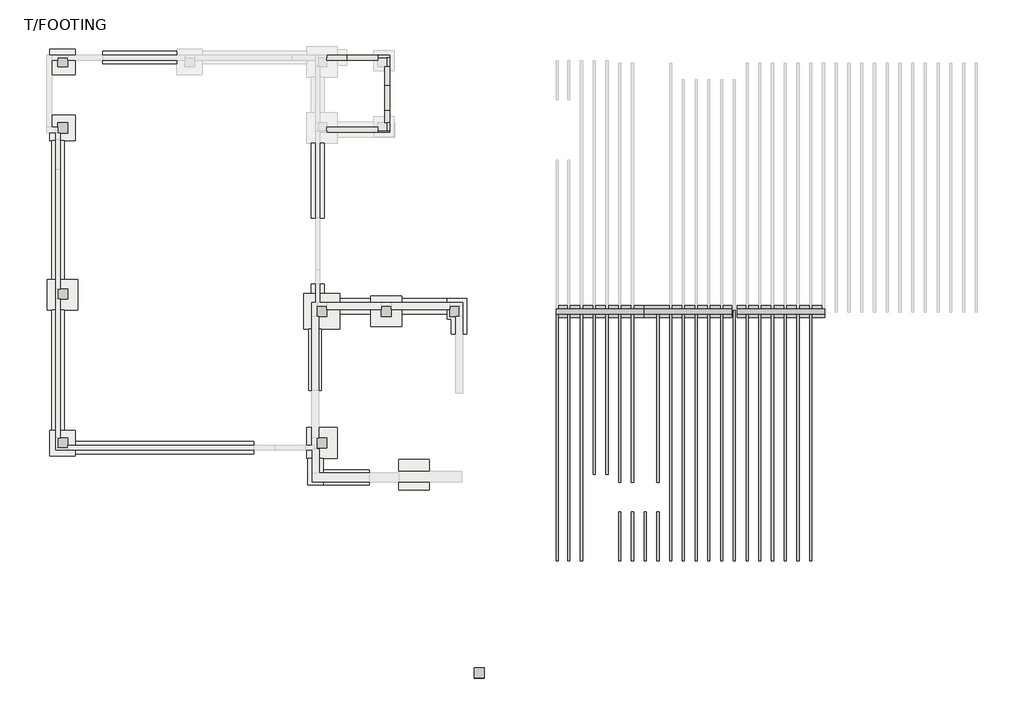
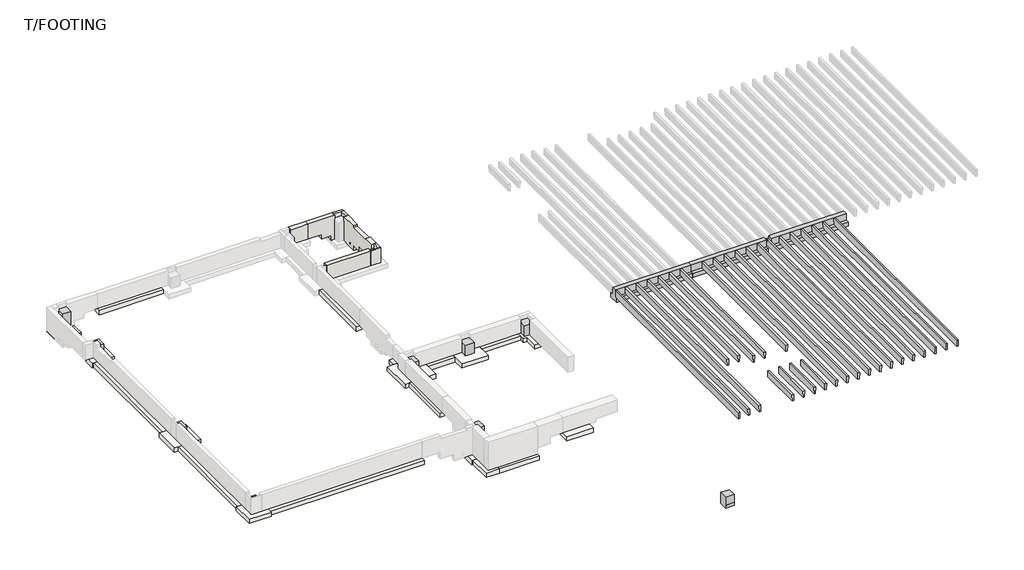
# One storey, part 2 of 3: 27 beams, 11 footings, 9 columns, 9 slabs, 8 walls.
"""IFC4 building model written with IfcOpenShell, lengths in millimetres."""

import ifcopenshell
import ifcopenshell.guid

model = None  # the IFC model being written
_history = None  # IfcOwnerHistory: only IFC2X3 demands one
_inside = {}  # id of a spatial element -> (the spatial element, [elements in it])
_under = {}  # id of a project, library or spatial element -> (it, [spatial elements below it])
_declared = {}  # id of a project -> (the project, [libraries it declares])
_typed = {}  # id of a type object -> (the type object, [elements of that type])
_made_of = {}  # id of a material, layer set ... -> (it, [elements and type objects made of it])


def new_model(schema):
    """Start an empty IFC model of exactly this schema.

    Asked for "IFC4X3", IfcOpenShell would pick the latest addendum, in which some entities
    have other attributes; the version numbers below select the first issue.
    IFC2X3 requires an IfcOwnerHistory on every rooted entity: one is made here for all.
    """
    global model, _history
    if schema == "IFC4X3":
        model = ifcopenshell.file(schema_version=(4, 3, 0, 0))
    else:
        model = ifcopenshell.file(schema=schema)
    _inside.clear()
    _under.clear()
    _declared.clear()
    _typed.clear()
    _made_of.clear()
    _history = None
    if model.schema == "IFC2X3":
        org = make("IfcOrganization", Name="unknown")
        user = make(
            "IfcPersonAndOrganization",
            ThePerson=make("IfcPerson", FamilyName="unknown"),
            TheOrganization=org,
        )
        app = make(
            "IfcApplication",
            ApplicationDeveloper=org,
            Version="unknown",
            ApplicationFullName="unknown",
            ApplicationIdentifier="unknown",
        )
        _history = make(
            "IfcOwnerHistory",
            OwningUser=user,
            OwningApplication=app,
            ChangeAction="ADDED",
            CreationDate=0,
        )
    return model


def make(cls, **values):
    """One entity of the class cls with the attributes given. An attribute that is None is left unset."""
    return model.create_entity(
        cls, **{name: value for name, value in values.items() if value is not None}
    )


def rooted(cls, **values):
    """An entity with a GlobalId (a new one), such as an element, a storey or a relation."""
    return make(cls, GlobalId=ifcopenshell.guid.new(), OwnerHistory=_history, **values)


def si_unit(unit_type, name, prefix=None):
    """IfcSIUnit, for example si_unit("LENGTHUNIT", "METRE", prefix="MILLI")."""
    return make("IfcSIUnit", UnitType=unit_type, Prefix=prefix, Name=name)


def assignment(units):
    """IfcUnitAssignment: the units of a project."""
    return None if units is None else make("IfcUnitAssignment", Units=units)


def point(xyz):
    """IfcCartesianPoint."""
    return None if xyz is None else make("IfcCartesianPoint", Coordinates=xyz)


def direction(xyz):
    """IfcDirection."""
    return None if xyz is None else make("IfcDirection", DirectionRatios=xyz)


def frame(location, z_axis=None, x_axis=None):
    """IfcAxis2Placement3D, a coordinate frame: its origin and axes. An axis left out is left unset."""
    return make(
        "IfcAxis2Placement3D",
        Location=point(location),
        Axis=direction(z_axis),
        RefDirection=direction(x_axis),
    )


def origin():
    """The frame at (0, 0, 0) with its axes left unset."""
    return frame((0.0, 0.0, 0.0))


def place(relative_to, where):
    """IfcLocalPlacement: puts the frame where relative to a parent placement (None: the world)."""
    return make(
        "IfcLocalPlacement", PlacementRelTo=relative_to, RelativePlacement=where
    )


def context(
    kind, dimensions, precision=None, world=None, true_north=None, identifier=None
):
    """IfcGeometricRepresentationContext, for example the 3D "Model" context."""
    return make(
        "IfcGeometricRepresentationContext",
        ContextIdentifier=identifier,
        ContextType=kind,
        CoordinateSpaceDimension=dimensions,
        Precision=precision,
        WorldCoordinateSystem=world,
        TrueNorth=true_north,
    )


def project(units=None, contexts=None):
    """IfcProject with its units and contexts."""
    return rooted(
        "IfcProject",
        Name="project",
        RepresentationContexts=contexts,
        UnitsInContext=assignment(units),
    )


def spatial(cls, under=None, at=None, **own):
    """A site, building, storey or space (cls), placed at a placement, below another one or the project."""
    s = rooted(cls, ObjectPlacement=at, **own)
    if under is not None:
        _under.setdefault(under.id(), (under, []))[1].append(s)
    return s


def polyline(points):
    """IfcPolyline through the points."""
    return make("IfcPolyline", Points=[point(p) for p in points])


def circle_curve(where, radius):
    """IfcCircle in the frame where."""
    return make("IfcCircle", Position=where, Radius=radius)


def outline(outer, holes=None, kind="AREA"):
    """IfcArbitraryClosedProfileDef: a profile drawn as a closed curve; with holes, ...WithVoids."""
    if holes is None:
        return make("IfcArbitraryClosedProfileDef", ProfileType=kind, OuterCurve=outer)
    return make(
        "IfcArbitraryProfileDefWithVoids",
        ProfileType=kind,
        OuterCurve=outer,
        InnerCurves=holes,
    )


def extrude(swept, where, along, depth):
    """IfcExtrudedAreaSolid: the profile swept, set in the frame where, extruded along a direction by depth."""
    return make(
        "IfcExtrudedAreaSolid",
        SweptArea=swept,
        Position=where,
        ExtrudedDirection=direction(along),
        Depth=depth,
    )


def faces_of(points, faces, orient=None, outer=None):
    """IfcFace entities. A face is a list of loops; a loop is a list of indices into points, from 0.

    orient and outer hold one flag for each loop. By default every Orientation is true, the
    first loop of a face is its IfcFaceOuterBound and the others are IfcFaceBound.
    """
    made = []
    for i, loops in enumerate(faces):
        bounds = []
        for j, loop in enumerate(loops):
            is_outer = j == 0 if outer is None else outer[i][j]
            bounds.append(
                make(
                    "IfcFaceOuterBound" if is_outer else "IfcFaceBound",
                    Bound=make("IfcPolyLoop", Polygon=[points[k] for k in loop]),
                    Orientation=True if orient is None else orient[i][j],
                )
            )
        made.append(make("IfcFace", Bounds=bounds))
    return made


def faceted_brep(points, faces, orient=None, outer=None, voids=None):
    """IfcFacetedBrep: a solid bounded by flat faces; with voids (closed shells), ...WithVoids."""
    shared = [point(p) for p in points]
    hull = make("IfcClosedShell", CfsFaces=faces_of(shared, faces, orient, outer))
    if voids is None:
        return make("IfcFacetedBrep", Outer=hull)
    return make(
        "IfcFacetedBrepWithVoids",
        Outer=hull,
        Voids=[
            make(cls, CfsFaces=faces_of(shared, fs, o, b)) for cls, fs, o, b in voids
        ],
    )


def shape(context_of_items, identifier, shape_type, items):
    """IfcShapeRepresentation: the items that make up one representation, for example the "Body"."""
    return make(
        "IfcShapeRepresentation",
        ContextOfItems=context_of_items,
        RepresentationIdentifier=identifier,
        RepresentationType=shape_type,
        Items=items,
    )


def source(mapping_origin, context_of_items, identifier, shape_type, items):
    """IfcRepresentationMap: a shape defined once, which mapped items show again and again."""
    return make(
        "IfcRepresentationMap",
        MappingOrigin=mapping_origin,
        MappedRepresentation=shape(context_of_items, identifier, shape_type, items),
    )


def transform(
    local_origin,
    x_axis=None,
    y_axis=None,
    z_axis=None,
    scale=None,
    scale2=None,
    scale3=None,
    uniform=True,
):
    """IfcCartesianTransformationOperator3D, or its non-uniform kind. x_axis, y_axis, z_axis: its Axis1, 2, 3."""
    if uniform:
        return make(
            "IfcCartesianTransformationOperator3D",
            Axis1=direction(x_axis),
            Axis2=direction(y_axis),
            LocalOrigin=point(local_origin),
            Scale=scale,
            Axis3=direction(z_axis),
        )
    return make(
        "IfcCartesianTransformationOperator3DnonUniform",
        Axis1=direction(x_axis),
        Axis2=direction(y_axis),
        LocalOrigin=point(local_origin),
        Scale=scale,
        Axis3=direction(z_axis),
        Scale2=scale2,
        Scale3=scale3,
    )


def mapped(mapping_source, mapping_target):
    """IfcMappedItem: shows the shape of a source again, moved by a transform."""
    return make(
        "IfcMappedItem", MappingSource=mapping_source, MappingTarget=mapping_target
    )


def made_of(thing, what):
    """Note that an element or type object is made of a material, layer set ...; save() writes the relation."""
    if what is not None:
        _made_of.setdefault(what.id(), (what, []))[1].append(thing)
    return thing


def element(
    cls,
    number,
    at=None,
    inside=None,
    cuts=None,
    type_object=None,
    material=None,
    context=None,
    identifier="Body",
    shape_type=None,
    held_by="IfcProductDefinitionShape",
    body=None,
    shapes=None,
    **own,
):
    """One element of the class cls, such as IfcWall. Its Tag is "e" and its number.

    at: its placement. inside: the storey or other place that contains it. cuts: it is an
    opening in that element (IfcRelVoidsElement). A single representation is given by context,
    identifier, shape_type and body (its items); several are given by shapes. held_by: the class
    of the entity that holds the representations. save() writes the other relations.
    """
    e = rooted(cls, Tag="e%d" % number, ObjectPlacement=at, **own)
    if body is not None:
        shapes = [shape(context, identifier, shape_type, body)]
    if shapes is not None:
        e.Representation = make(held_by, Representations=shapes)
    if inside is not None:
        _inside.setdefault(inside.id(), (inside, []))[1].append(e)
    if cuts is not None:
        rooted(
            "IfcRelVoidsElement", RelatingBuildingElement=cuts, RelatedOpeningElement=e
        )
    if type_object is not None:
        _typed.setdefault(type_object.id(), (type_object, []))[1].append(e)
    return made_of(e, material)


def aggregate(whole, parts):
    """IfcRelAggregates: a whole, such as a stair, and the parts it consists of."""
    return rooted("IfcRelAggregates", RelatingObject=whole, RelatedObjects=parts)


def save(model, path):
    """Write the relations noted so far, then the file.

    IfcRelAggregates (storeys below a building ...), IfcRelContainedInSpatialStructure (elements
    in a storey), IfcRelDefinesByType, IfcRelAssociatesMaterial and IfcRelDeclares: one each for
    every whole, place, type object, material and project.
    """
    for whole, parts in _under.values():
        aggregate(whole, parts)
    for where, things in _inside.values():
        rooted(
            "IfcRelContainedInSpatialStructure",
            RelatedElements=things,
            RelatingStructure=where,
        )
    for kind, things in _typed.values():
        rooted("IfcRelDefinesByType", RelatedObjects=things, RelatingType=kind)
    for what, things in _made_of.values():
        rooted("IfcRelAssociatesMaterial", RelatedObjects=things, RelatingMaterial=what)
    for by, libraries in _declared.values():
        rooted("IfcRelDeclares", RelatingContext=by, RelatedDefinitions=libraries)
    model.write(path)


def plane_surface(at):
    """IfcPlane: the flat surface through the origin of the frame at, square to its z axis."""
    return make("IfcPlane", Position=at)


def revolved_surface(curve, axis_point, axis_direction):
    """IfcSurfaceOfRevolution: the curve turned about the line through axis_point along axis_direction."""
    return make(
        "IfcSurfaceOfRevolution",
        SweptCurve=make("IfcArbitraryOpenProfileDef", ProfileType="CURVE", Curve=curve),
        AxisPosition=make("IfcAxis1Placement", Location=point(axis_point), Axis=direction(axis_direction)),
    )


def advanced_brep(points, edges, surfaces, faces):
    """IfcAdvancedBrep: a solid bounded by faces that lie on surfaces and meet in shared edges.

    An edge is (start, end): straight between two places in points (the first is 0);
    or (start, end, curve); or (start, end, curve, False) where it runs against its curve.
    A face is (place in surfaces, loops), or (place, loops, False) where it looks against
    its surface's normal. A loop lists edges by number (the first is 1), with a minus sign
    where the edge is run from its end to its start. The first loop is the outer one.
    """
    corners = [point(p) for p in points]
    vertices = [make("IfcVertexPoint", VertexGeometry=c) for c in corners]
    made = []
    for start, end, *more in edges:
        made.append(
            make(
                "IfcEdgeCurve",
                EdgeStart=vertices[start],
                EdgeEnd=vertices[end],
                EdgeGeometry=more[0] if more else make("IfcPolyline", Points=[corners[start], corners[end]]),
                SameSense=more[1] if len(more) > 1 else True,
            )
        )
    hull = []
    for where, loops, *sense in faces:
        bounds = []
        for j, loop in enumerate(loops):
            ring = [make("IfcOrientedEdge", EdgeElement=made[abs(k) - 1], Orientation=k > 0) for k in loop]
            bounds.append(
                make(
                    "IfcFaceOuterBound" if j == 0 else "IfcFaceBound",
                    Bound=make("IfcEdgeLoop", EdgeList=ring),
                    Orientation=True,
                )
            )
        hull.append(make("IfcAdvancedFace", Bounds=bounds, FaceSurface=surfaces[where], SameSense=sense[0] if sense else True))
    return make("IfcAdvancedBrep", Outer=make("IfcClosedShell", CfsFaces=hull))


def precast_cone_shaped_beam_double_t_64f85e83(model_context):
    return source(origin(), model_context, "Body", "SweptSolid", [
        extrude(outline(polyline([(-50.8, -228.6), (-63.5, 228.6), (63.5, 228.6), (50.8, -228.6), (-50.8, -228.6)])), frame((-7391.4, 0.0, 0.0), z_axis=(1.0, 0.0, 0.0), x_axis=(0.0, 1.0, 0.0)), (0.0, 0.0, 1.0), 14770.1),
    ])


def precast_cone_shaped_beam_double_t_17914b82(model_context):
    return source(origin(), model_context, "Body", "SweptSolid", [
        extrude(outline(polyline([(-50.8, -228.6), (-63.5, 228.6), (63.5, 228.6), (50.8, -228.6), (-50.8, -228.6)])), frame((-7594.6, 0.0, 0.0), z_axis=(1.0, 0.0, 0.0), x_axis=(0.0, 1.0, 0.0)), (0.0, 0.0, 1.0), 14973.3),
    ])


def precast_cone_shaped_beam_double_t_a1b90a55(model_context):
    return source(origin(), model_context, "Body", "SweptSolid", [
        extrude(outline(polyline([(-50.8, -228.6), (-63.5, 228.6), (63.5, 228.6), (50.8, -228.6), (-50.8, -228.6)])), frame((-4891.88125, 0.0, 0.0), z_axis=(1.0, 0.0, 0.0), x_axis=(0.0, 1.0, 0.0)), (0.0, 0.0, 1.0), 10083.8),
    ])


def precast_cone_shaped_beam_double_t_8ba99103(model_context):
    return source(origin(), model_context, "Body", "SweptSolid", [
        extrude(outline(polyline([(50.8, -228.6), (-50.8, -228.6), (-63.5, 228.6), (63.5, 228.6), (50.8, -228.6)])), frame((-1610.51875, 0.0, 0.0), z_axis=(1.0, 0.0, 0.0), x_axis=(0.0, 1.0, 0.0)), (0.0, 0.0, 1.0), 2908.3),
    ])


def precast_cone_shaped_beam_double_t_5ff23cd5(model_context):
    return source(origin(), model_context, "Body", "SweptSolid", [
        extrude(outline(polyline([(-50.8, -228.6), (-63.5, 228.6), (63.5, 228.6), (50.8, -228.6), (-50.8, -228.6)])), frame((-4660.9, 0.0, 0.0), z_axis=(1.0, 0.0, 0.0), x_axis=(0.0, 1.0, 0.0)), (0.0, 0.0, 1.0), 9601.2),
    ])


def precast_inverted_tee_20_12x28_77df7164(model_context):
    return source(origin(), model_context, "Body", "SweptSolid", [
        extrude(outline(polyline([(-355.6, -406.4), (-355.6, -101.6), (-152.4, -101.6), (-152.4, 406.4), (152.4, 406.4), (152.4, -101.6), (355.6, -101.6), (355.6, -406.4), (-355.6, -406.4)])), frame((-2728.5280327, 0.0, 0.0), z_axis=(1.0, 0.0, 0.0), x_axis=(0.0, 1.0, 0.0)), (0.0, 0.0, 1.0), 5228.4560654),
    ])


def precast_inverted_tee_20_12x28_0a739a6f(model_context):
    return source(origin(), model_context, "Body", "SweptSolid", [
        extrude(outline(polyline([(355.6, -406.4), (-355.6, -406.4), (-355.6, -101.6), (-152.4, -101.6), (-152.4, 406.4), (152.4, 406.4), (152.4, -101.6), (355.6, -101.6), (355.6, -406.4)])), frame((-2692.4, 0.0, 0.0), z_axis=(1.0, 0.0, 0.0), x_axis=(0.0, 1.0, 0.0)), (0.0, 0.0, 1.0), 5245.1),
    ])


def precast_inverted_tee_20_12x28_b7649b98(model_context):
    return source(origin(), model_context, "Body", "SweptSolid", [
        extrude(outline(polyline([(355.6, -406.4), (-355.6, -406.4), (-355.6, -101.6), (-152.4, -101.6), (-152.4, 406.4), (152.4, 406.4), (152.4, -101.6), (355.6, -101.6), (355.6, -406.4)])), frame((-2730.5, 0.0, 0.0), z_axis=(1.0, 0.0, 0.0), x_axis=(0.0, 1.0, 0.0)), (0.0, 0.0, 1.0), 5232.4),
    ])


model = new_model("IFC4")

# Units and contexts
model_context = context("Model", 3, world=origin())
ifc_project = project(units=[si_unit("LENGTHUNIT", "METRE", prefix="MILLI")], contexts=[model_context])

# Site, building, storey
site = spatial("IfcSite", under=ifc_project)
building = spatial("IfcBuilding", under=site)
storey = spatial("IfcBuildingStorey", under=building, Name="T/FOOTING", Elevation=-1092.2)

# Beams
placement = place(None, origin())
precast_cone_shaped_beam_double_t_shape = precast_cone_shaped_beam_double_t_64f85e83(model_context)
element("IfcBeam", 1, ObjectType="Precast-Cone Shaped Beam : DOUBLE_T", at=placement, inside=storey, context=model_context, shape_type="MappedRepresentation", body=[
    mapped(precast_cone_shaped_beam_double_t_shape, transform((-28033.5909443, -9707.8231529, -279.4), x_axis=(0.0, -1.0, 0.0), y_axis=(1.0, 0.0, 0.0), z_axis=(0.0, 0.0, 1.0))),
])
element("IfcBeam", 2, ObjectType="Precast-Cone Shaped Beam : DOUBLE_T", at=placement, inside=storey, context=model_context, shape_type="MappedRepresentation", body=[
    mapped(precast_cone_shaped_beam_double_t_shape, transform((-27271.5909443, -9707.8231529, -279.4), x_axis=(0.0, -1.0, 0.0), y_axis=(1.0, 0.0, 0.0), z_axis=(0.0, 0.0, 1.0))),
])
element("IfcBeam", 3, ObjectType="Precast-Cone Shaped Beam : DOUBLE_T", at=placement, inside=storey, context=model_context, shape_type="MappedRepresentation", body=[
    mapped(precast_cone_shaped_beam_double_t_shape, transform((-26509.5909443, -9707.8231529, -279.4), x_axis=(0.0, -1.0, 0.0), y_axis=(1.0, 0.0, 0.0), z_axis=(0.0, 0.0, 1.0))),
])
element("IfcBeam", 4, ObjectType="Precast-Cone Shaped Beam : DOUBLE_T", at=placement, inside=storey, context=model_context, shape_type="MappedRepresentation", body=[
    mapped(precast_cone_shaped_beam_double_t_shape, transform((-25747.5909443, -9707.8231529, -279.4), x_axis=(0.0, -1.0, 0.0), y_axis=(1.0, 0.0, 0.0), z_axis=(0.0, 0.0, 1.0))),
])
element("IfcBeam", 5, ObjectType="Precast-Cone Shaped Beam : DOUBLE_T", at=placement, inside=storey, context=model_context, shape_type="MappedRepresentation", body=[
    mapped(precast_cone_shaped_beam_double_t_shape, transform((-24985.5909443, -9707.8231529, -279.4), x_axis=(0.0, -1.0, 0.0), y_axis=(1.0, 0.0, 0.0), z_axis=(0.0, 0.0, 1.0))),
])
element("IfcBeam", 6, ObjectType="Precast-Cone Shaped Beam : DOUBLE_T", at=placement, inside=storey, context=model_context, shape_type="MappedRepresentation", body=[
    mapped(precast_cone_shaped_beam_double_t_shape, transform((-23461.5909443, -9707.8231529, -279.4), x_axis=(0.0, -1.0, 0.0), y_axis=(1.0, 0.0, 0.0), z_axis=(0.0, 0.0, 1.0))),
])
element("IfcBeam", 7, ObjectType="Precast-Cone Shaped Beam : DOUBLE_T", at=placement, inside=storey, context=model_context, shape_type="MappedRepresentation", body=[
    mapped(precast_cone_shaped_beam_double_t_shape, transform((-22699.5909443, -9707.8231529, -279.4), x_axis=(0.0, -1.0, 0.0), y_axis=(1.0, 0.0, 0.0), z_axis=(0.0, 0.0, 1.0))),
])
element("IfcBeam", 8, ObjectType="Precast-Cone Shaped Beam : DOUBLE_T", at=placement, inside=storey, context=model_context, shape_type="MappedRepresentation", body=[
    mapped(precast_cone_shaped_beam_double_t_shape, transform((-21940.4905844, -9707.8231529, -279.4), x_axis=(0.0, -1.0, 0.0), y_axis=(1.0, 0.0, 0.0), z_axis=(0.0, 0.0, 1.0))),
])
element("IfcBeam", 9, ObjectType="Precast-Cone Shaped Beam : DOUBLE_T", at=placement, inside=storey, context=model_context, shape_type="MappedRepresentation", body=[
    mapped(precast_cone_shaped_beam_double_t_shape, transform((-21179.5348789, -9707.8231529, -279.4), x_axis=(0.0, -1.0, 0.0), y_axis=(1.0, 0.0, 0.0), z_axis=(0.0, 0.0, 1.0))),
])
element("IfcBeam", 10, ObjectType="Precast-Cone Shaped Beam : DOUBLE_T", at=placement, inside=storey, context=model_context, shape_type="MappedRepresentation", body=[
    mapped(precast_cone_shaped_beam_double_t_shape, transform((-20417.5348789, -9707.8231529, -279.4), x_axis=(0.0, -1.0, 0.0), y_axis=(1.0, 0.0, 0.0), z_axis=(0.0, 0.0, 1.0))),
])
element("IfcBeam", 11, ObjectType="Precast-Cone Shaped Beam : DOUBLE_T", at=placement, inside=storey, context=model_context, shape_type="MappedRepresentation", body=[
    mapped(precast_cone_shaped_beam_double_t_shape, transform((-19655.5348789, -9707.8231529, -279.4), x_axis=(0.0, -1.0, 0.0), y_axis=(1.0, 0.0, 0.0), z_axis=(0.0, 0.0, 1.0))),
])
element("IfcBeam", 12, ObjectType="Precast-Cone Shaped Beam : DOUBLE_T", at=placement, inside=storey, context=model_context, shape_type="MappedRepresentation", body=[
    mapped(precast_cone_shaped_beam_double_t_shape, transform((-33367.5909443, -9707.8231529, -279.4), x_axis=(0.0, -1.0, 0.0), y_axis=(1.0, 0.0, 0.0), z_axis=(0.0, 0.0, 1.0))),
])
element("IfcBeam", 13, ObjectType="Precast-Cone Shaped Beam : DOUBLE_T", at=placement, inside=storey, context=model_context, shape_type="MappedRepresentation", body=[
    mapped(precast_cone_shaped_beam_double_t_shape, transform((-34129.5909443, -9707.8231529, -279.4), x_axis=(0.0, -1.0, 0.0), y_axis=(1.0, 0.0, 0.0), z_axis=(0.0, 0.0, 1.0))),
])
element("IfcBeam", 14, ObjectType="Precast-Cone Shaped Beam : DOUBLE_T", at=placement, inside=storey, context=model_context, shape_type="MappedRepresentation", body=[
    mapped(precast_cone_shaped_beam_double_t_shape, transform((-34815.3909443, -9707.8231529, -279.4), x_axis=(0.0, -1.0, 0.0), y_axis=(1.0, 0.0, 0.0), z_axis=(0.0, 0.0, 1.0))),
])
precast_cone_shaped_beam_double_t_2_shape = precast_cone_shaped_beam_double_t_17914b82(model_context)
element("IfcBeam", 15, ObjectType="Precast-Cone Shaped Beam : DOUBLE_T", at=placement, inside=storey, context=model_context, shape_type="MappedRepresentation", body=[
    mapped(precast_cone_shaped_beam_double_t_2_shape, transform((-24223.5909443, -9707.8231529, -279.4), x_axis=(0.0, -1.0, 0.0), y_axis=(1.0, 0.0, 0.0), z_axis=(0.0, 0.0, 1.0))),
])
precast_cone_shaped_beam_double_t_3_shape = precast_cone_shaped_beam_double_t_a1b90a55(model_context)
element("IfcBeam", 16, ObjectType="Precast-Cone Shaped Beam : DOUBLE_T", at=placement, inside=storey, context=model_context, shape_type="MappedRepresentation", body=[
    mapped(precast_cone_shaped_beam_double_t_3_shape, transform((-28795.5909443, -7208.3044029, -279.4), x_axis=(0.0, -1.0, 0.0), y_axis=(1.0, 0.0, 0.0), z_axis=(0.0, 0.0, 1.0))),
])
element("IfcBeam", 17, ObjectType="Precast-Cone Shaped Beam : DOUBLE_T", at=placement, inside=storey, context=model_context, shape_type="MappedRepresentation", body=[
    mapped(precast_cone_shaped_beam_double_t_3_shape, transform((-30319.5909443, -7208.3044029, -279.4), x_axis=(0.0, -1.0, 0.0), y_axis=(1.0, 0.0, 0.0), z_axis=(0.0, 0.0, 1.0))),
])
element("IfcBeam", 18, ObjectType="Precast-Cone Shaped Beam : DOUBLE_T", at=placement, inside=storey, context=model_context, shape_type="MappedRepresentation", body=[
    mapped(precast_cone_shaped_beam_double_t_3_shape, transform((-31081.5909443, -7208.3044029, -279.4), x_axis=(0.0, -1.0, 0.0), y_axis=(1.0, 0.0, 0.0), z_axis=(0.0, 0.0, 1.0))),
])
precast_cone_shaped_beam_double_t_4_shape = precast_cone_shaped_beam_double_t_8ba99103(model_context)
element("IfcBeam", 19, ObjectType="Precast-Cone Shaped Beam : DOUBLE_T", at=placement, inside=storey, context=model_context, shape_type="MappedRepresentation", body=[
    mapped(precast_cone_shaped_beam_double_t_4_shape, transform((-28795.5909443, -15788.7419029, -279.4), x_axis=(0.0, -1.0, 0.0), y_axis=(1.0, 0.0, 0.0), z_axis=(0.0, 0.0, 1.0))),
])
element("IfcBeam", 20, ObjectType="Precast-Cone Shaped Beam : DOUBLE_T", at=placement, inside=storey, context=model_context, shape_type="MappedRepresentation", body=[
    mapped(precast_cone_shaped_beam_double_t_4_shape, transform((-30319.5909443, -15788.7419029, -279.4), x_axis=(0.0, -1.0, 0.0), y_axis=(1.0, 0.0, 0.0), z_axis=(0.0, 0.0, 1.0))),
])
element("IfcBeam", 21, ObjectType="Precast-Cone Shaped Beam : DOUBLE_T", at=placement, inside=storey, context=model_context, shape_type="MappedRepresentation", body=[
    mapped(precast_cone_shaped_beam_double_t_4_shape, transform((-31081.5909443, -15788.7419029, -279.4), x_axis=(0.0, -1.0, 0.0), y_axis=(1.0, 0.0, 0.0), z_axis=(0.0, 0.0, 1.0))),
])
element("IfcBeam", 22, ObjectType="Precast-Cone Shaped Beam : DOUBLE_T", at=placement, inside=storey, context=model_context, shape_type="MappedRepresentation", body=[
    mapped(precast_cone_shaped_beam_double_t_4_shape, transform((-29557.5909443, -15788.7419029, -279.4), x_axis=(0.0, -1.0, 0.0), y_axis=(1.0, 0.0, 0.0), z_axis=(0.0, 0.0, 1.0))),
])
precast_cone_shaped_beam_double_t_5_shape = precast_cone_shaped_beam_double_t_5ff23cd5(model_context)
element("IfcBeam", 23, ObjectType="Precast-Cone Shaped Beam : DOUBLE_T", at=placement, inside=storey, context=model_context, shape_type="MappedRepresentation", body=[
    mapped(precast_cone_shaped_beam_double_t_5_shape, transform((-31843.5909443, -6977.3231529, -279.4), x_axis=(0.0, -1.0, 0.0), y_axis=(1.0, 0.0, 0.0), z_axis=(0.0, 0.0, 1.0))),
])
element("IfcBeam", 24, ObjectType="Precast-Cone Shaped Beam : DOUBLE_T", at=placement, inside=storey, context=model_context, shape_type="MappedRepresentation", body=[
    mapped(precast_cone_shaped_beam_double_t_5_shape, transform((-32605.5909443, -6977.3231529, -279.4), x_axis=(0.0, -1.0, 0.0), y_axis=(1.0, 0.0, 0.0), z_axis=(0.0, 0.0, 1.0))),
])
precast_inverted_tee_20_12x28_shape = precast_inverted_tee_20_12x28_77df7164(model_context)
element("IfcBeam", 25, ObjectType="Precast-Inverted Tee : 20+12X28", at=placement, inside=storey, context=model_context, shape_type="MappedRepresentation", body=[
    mapped(precast_inverted_tee_20_12x28_shape, transform((-21558.5629116, -2164.0231529, -406.4), x_axis=(-1.0, 0.0, 0.0), y_axis=(0.0, -1.0, 0.0), z_axis=(0.0, 0.0, 1.0))),
])
precast_inverted_tee_20_12x28_2_shape = precast_inverted_tee_20_12x28_0a739a6f(model_context)
element("IfcBeam", 26, ObjectType="Precast-Inverted Tee : 20+12X28", at=placement, inside=storey, context=model_context, shape_type="MappedRepresentation", body=[
    mapped(precast_inverted_tee_20_12x28_2_shape, transform((-32186.4909443, -2164.0231529, -406.4), x_axis=(1.0, 0.0, 0.0), y_axis=(0.0, 1.0, 0.0), z_axis=(0.0, 0.0, 1.0))),
])
precast_inverted_tee_20_12x28_3_shape = precast_inverted_tee_20_12x28_b7649b98(model_context)
element("IfcBeam", 27, ObjectType="Precast-Inverted Tee : 20+12X28", at=placement, inside=storey, context=model_context, shape_type="MappedRepresentation", body=[
    mapped(precast_inverted_tee_20_12x28_3_shape, transform((-26890.5909443, -2164.0231529, -406.4), x_axis=(1.0, 0.0, 0.0), y_axis=(0.0, 1.0, 0.0), z_axis=(0.0, 0.0, 1.0))),
])

# Columns
element("IfcColumn", 28, ObjectType="Concrete-Square-Column : PIER 24\"x24\"", at=placement, inside=storey, context=model_context, shape_type="Brep", body=[
    faceted_brep([(-41257.5850821, -2468.8231529, -1092.2), (-41257.5850821, -2062.4231529, -1092.2), (-41257.5850821, -1859.2231529, -1092.2), (-40686.0850821, -1859.2231529, -1092.2), (-40686.0850821, -2468.8231529, -1092.2), (-40901.9850821, -2468.8231529, -1092.2), (-41257.5850821, -2468.8231529, -304.8), (-40686.0850821, -2468.8231529, -304.8), (-41257.5850821, -1859.2231529, -304.8), (-40686.0850821, -1859.2231529, -304.8)], [[[0, 1, 2, 3, 4, 5]], [[6, 0, 5, 4, 7]], [[2, 1, 0, 6, 8]], [[2, 8, 9, 3]], [[8, 6, 7, 9]], [[4, 3, 9, 7]]]),
])
element("IfcColumn", 29, ObjectType="Concrete-Square-Column : PIER 24\"x24\"", at=placement, inside=storey, context=model_context, shape_type="Brep", body=[
    faceted_brep([(-44741.4490821, -1859.2231529, -1092.2), (-44741.4490821, -2062.4231529, -1092.2), (-44741.4490821, -2468.8231529, -1092.2), (-45351.0490821, -2468.8231529, -1092.2), (-45351.0490821, -2062.4231529, -1092.2), (-45351.0490821, -1859.2231529, -1092.2), (-44741.4490821, -1859.2231529, -304.8), (-44741.4490821, -2468.8231529, -304.8), (-45351.0490821, -2468.8231529, -304.8), (-45351.0490821, -1859.2231529, -304.8)], [[[0, 1, 2, 3, 4, 5]], [[6, 7, 2, 1, 0]], [[7, 8, 3, 2]], [[8, 9, 5, 4, 3]], [[9, 6, 0, 5]], [[6, 9, 8, 7]]]),
])
element("IfcColumn", 30, ObjectType="Concrete-Square-Column : PIER 24\"x24\"", at=placement, inside=storey, context=model_context, shape_type="Brep", body=[
    faceted_brep([(-48601.3600821, -1859.2231529, -1092.2), (-48601.3600821, -2468.8231529, -1092.2), (-49093.4850821, -2468.8231529, -1092.2), (-49207.7850821, -2468.8231529, -1092.2), (-49207.7850821, -1859.2231529, -1092.2), (-48601.3600821, -1859.2231529, -304.8), (-48601.3600821, -2468.8231529, -304.8), (-49207.7850821, -2468.8231529, -304.8), (-49207.7850821, -1859.2231529, -304.8)], [[[0, 1, 2, 3, 4]], [[1, 0, 5, 6]], [[1, 6, 7, 3, 2]], [[5, 0, 4, 8]], [[6, 5, 8, 7]], [[4, 3, 7, 8]]]),
])
element("IfcColumn", 31, ObjectType="Concrete-Square-Column : PIER 24\"x24\"", at=placement, inside=storey, context=model_context, shape_type="Brep", body=[
    faceted_brep([(-48601.3600821, -9733.2231529, -2057.4), (-48601.3600821, -10342.8231529, -2057.4), (-49207.7850821, -10342.8231529, -2057.4), (-49207.7850821, -9733.2231529, -2057.4), (-49093.4850821, -9733.2231529, -2057.4), (-48601.3600821, -9733.2231529, -304.8), (-48601.3600821, -10342.8231529, -304.8), (-49207.7850821, -10342.8231529, -304.8), (-49207.7850821, -9733.2231529, -304.8)], [[[0, 1, 2, 3, 4]], [[1, 0, 5, 6]], [[1, 6, 7, 2]], [[5, 0, 4, 3, 8]], [[6, 5, 8, 7]], [[3, 2, 7, 8]]]),
])
element("IfcColumn", 32, ObjectType="Concrete-Square-Column : PIER 24\"x24\"", at=placement, inside=storey, context=model_context, shape_type="Brep", body=[
    faceted_brep([(-64092.1850821, -9733.2231529, -1092.2), (-64092.1850821, -10190.4231529, -1092.2), (-64092.1850821, -10342.8231529, -1092.2), (-64701.7850821, -10342.8231529, -1092.2), (-64701.7850821, -9733.2231529, -1092.2), (-64549.3850821, -9733.2231529, -1092.2), (-64092.1850821, -9733.2231529, -304.8), (-64092.1850821, -10342.8231529, -304.8), (-64701.7850821, -10342.8231529, -304.8), (-64701.7850821, -9733.2231529, -304.8)], [[[0, 1, 2, 3, 4, 5]], [[6, 7, 2, 1, 0]], [[7, 8, 3, 2]], [[8, 9, 4, 3]], [[9, 6, 0, 5, 4]], [[6, 9, 8, 7]]]),
])
element("IfcColumn", 33, ObjectType="Concrete-Square-Column : PIER 24\"x24\"", at=placement, inside=storey, context=model_context, shape_type="Brep", body=[
    faceted_brep([(-64092.1850821, -826.5544032, -1092.2), (-64092.1850821, -1436.1544032, -1092.2), (-64549.3850821, -1436.1544032, -1092.2), (-64701.7850821, -1436.1544032, -1092.2), (-64701.7850821, -826.5544032, -1092.2), (-64549.3850821, -826.5544032, -1092.2), (-64092.1850821, -826.5544032, -304.8), (-64092.1850821, -1436.1544032, -304.8), (-64701.7850821, -1436.1544032, -304.8), (-64701.7850821, -826.5544032, -304.8)], [[[0, 1, 2, 3, 4, 5]], [[6, 7, 1, 0]], [[7, 8, 3, 2, 1]], [[8, 9, 4, 3]], [[9, 6, 0, 5, 4]], [[6, 9, 8, 7]]]),
])
element("IfcColumn", 34, ObjectType="Concrete-Square-Column : PIER 24\"x24\"", at=placement, inside=storey, context=model_context, shape_type="Brep", body=[
    faceted_brep([(-64092.1850821, 9117.3505048, -1092.2), (-64092.1850821, 8507.7505048, -1092.2), (-64549.3850821, 8507.7505048, -1092.2), (-64701.7850821, 8507.7505048, -1092.2), (-64701.7850821, 8850.6505048, -1092.2), (-64701.7850821, 9117.3505048, -1092.2), (-64092.1850821, 9117.3505048, -304.8), (-64092.1850821, 8507.7505048, -304.8), (-64701.7850821, 8507.7505048, -304.8), (-64701.7850821, 9117.3505048, -304.8)], [[[0, 1, 2, 3, 4, 5]], [[6, 7, 1, 0]], [[7, 8, 3, 2, 1]], [[8, 9, 5, 4, 3]], [[9, 6, 0, 5]], [[6, 9, 8, 7]]]),
])
element("IfcColumn", 35, ObjectType="Concrete-Square-Column : PIER 24\"x24\"", at=placement, inside=storey, context=model_context, shape_type="Brep", body=[
    faceted_brep([(-64092.1850821, 12470.1505048, -1752.6), (-64701.7850821, 12470.1505048, -1752.6), (-64701.7850821, 12876.5505048, -1752.6), (-64701.7850821, 13028.9505048, -1752.6), (-64092.1850821, 13028.9505048, -1752.6), (-64092.1850821, 12470.1505048, -304.8), (-64092.1850821, 13028.9505048, -304.8), (-64701.7850821, 12470.1505048, -304.8), (-64701.7850821, 13028.9505048, -304.8)], [[[0, 1, 2, 3, 4]], [[5, 0, 4, 6]], [[1, 0, 5, 7]], [[1, 7, 8, 3, 2]], [[7, 5, 6, 8]], [[4, 3, 8, 6]]]),
])
element("IfcColumn", 36, ObjectType="Concrete-Square-Column : PIER 24\"x24\"", at=placement, inside=storey, context=model_context, shape_type="SweptSolid", body=[
    extrude(outline(polyline([(-23500.0231529, -1092.2), (-24109.6231529, -1092.2), (-24109.6231529, -863.6), (-24096.9231529, -863.6), (-24096.9231529, -304.8), (-23500.0231529, -304.8), (-23500.0231529, -1092.2)])), frame((-39790.6159443, 0.0, 0.0), z_axis=(1.0, 0.0, 0.0), x_axis=(0.0, 1.0, 0.0)), (0.0, 0.0, 1.0), 609.6),
])

# Footings
element("IfcFooting", 37, ObjectType="F4", at=placement, inside=storey, context=model_context, shape_type="Brep", body=[
    faceted_brep([(-49725.3100821, -12551.0356529, -2057.4), (-48810.9100821, -12551.0356529, -2057.4), (-48810.9100821, -11636.6356529, -2057.4), (-48810.9100821, -10952.4231529, -2057.4), (-49725.3100821, -10952.4231529, -2057.4), (-49725.3100821, -12551.0356529, -2362.2), (-49725.3100821, -10952.4231529, -2362.2), (-48810.9100821, -12551.0356529, -2362.2), (-48810.9100821, -10952.4231529, -2362.2), (-48810.9100821, -11636.6356529, -2362.2)], [[[0, 1, 2, 3, 4]], [[5, 0, 4, 6]], [[7, 5, 6, 8, 9]], [[1, 7, 9, 8, 3, 2]], [[1, 0, 5, 7]], [[4, 3, 8, 6]]]),
])
element("IfcFooting", 38, ObjectType="F4", at=placement, inside=storey, context=model_context, shape_type="SweptSolid", body=[
    extrude(outline(polyline([(-44131.8490821, -2310.0731529), (-44131.8490821, -1395.6731529), (-41409.9850821, -1395.6731529), (-41409.9850821, -2310.0731529), (-44131.8490821, -2310.0731529)])), frame((0.0, 0.0, -1397.0), z_axis=(0.0, 0.0, 1.0), x_axis=(1.0, 0.0, 0.0)), (0.0, 0.0, 1.0), 304.8),
])
element("IfcFooting", 39, ObjectType="F4", at=placement, inside=storey, context=model_context, shape_type="SweptSolid", body=[
    extrude(outline(polyline([(-47833.0100821, -2310.0731529), (-47833.0100821, -1395.6731529), (-45960.6490821, -1395.6731529), (-45960.6490821, -2310.0731529), (-47833.0100821, -2310.0731529)])), frame((0.0, 0.0, -1397.0), z_axis=(0.0, 0.0, 1.0), x_axis=(1.0, 0.0, 0.0)), (0.0, 0.0, 1.0), 304.8),
])
element("IfcFooting", 40, ObjectType="F4", at=placement, inside=storey, context=model_context, shape_type="SweptSolid", body=[
    extrude(outline(polyline([(-46055.0100821, -11636.6356529), (-46055.0100821, -12551.0356529), (-48810.9100821, -12551.0356529), (-48810.9100821, -11636.6356529), (-46055.0100821, -11636.6356529)])), frame((0.0, 0.0, -2362.2), z_axis=(0.0, 0.0, 1.0), x_axis=(1.0, 0.0, 0.0)), (0.0, 0.0, 1.0), 304.8),
])
element("IfcFooting", 41, ObjectType="WF_30IN", at=placement, inside=storey, context=model_context, shape_type="SweptSolid", body=[
    extrude(outline(polyline([(-65057.3850821, -2087.8231532), (-64295.3850821, -2087.8231532), (-64295.3850821, -9276.0231529), (-65057.3850821, -9276.0231529), (-65057.3850821, -2087.8231532)])), frame((0.0, 0.0, -1397.0), z_axis=(0.0, 0.0, 1.0), x_axis=(1.0, 0.0, 0.0)), (0.0, 0.0, 1.0), 304.8),
])
element("IfcFooting", 42, ObjectType="WF_30IN", at=placement, inside=storey, context=model_context, shape_type="SweptSolid", body=[
    extrude(outline(polyline([(-49515.7600821, -538.4231529), (-48753.7600821, -538.4231529), (-48753.7600821, -1097.2231529), (-49515.7600821, -1097.2231529), (-49515.7600821, -538.4231529)])), frame((0.0, 0.0, -1397.0), z_axis=(0.0, 0.0, 1.0), x_axis=(1.0, 0.0, 0.0)), (0.0, 0.0, 1.0), 304.8),
])
element("IfcFooting", 43, ObjectType="WF_30IN", at=placement, inside=storey, context=model_context, shape_type="SweptSolid", body=[
    extrude(outline(polyline([(-64295.3850821, -259.0231532), (-65057.3850821, -259.0231532), (-65057.3850821, 8050.5505048), (-64295.3850821, 8050.5505048), (-64295.3850821, -259.0231532)])), frame((0.0, 0.0, -1397.0), z_axis=(0.0, 0.0, 1.0), x_axis=(1.0, 0.0, 0.0)), (0.0, 0.0, 1.0), 304.8),
])
element("IfcFooting", 44, ObjectType="WF_30IN", at=placement, inside=storey, context=model_context, shape_type="SweptSolid", body=[
    extrude(outline(polyline([(-62009.3850821, 12647.9505048), (-62009.3850821, 13409.9505048), (-57564.3850821, 13409.9505048), (-57564.3850821, 12647.9505048), (-62009.3850821, 12647.9505048)])), frame((0.0, 0.0, -1397.0), z_axis=(0.0, 0.0, 1.0), x_axis=(1.0, 0.0, 0.0)), (0.0, 0.0, 1.0), 304.8),
])
element("IfcFooting", 45, ObjectType="WF_30IN", at=placement, inside=storey, context=model_context, shape_type="SweptSolid", body=[
    extrude(outline(polyline([(-48753.7600821, 3423.9768471), (-49515.7600821, 3423.9768471), (-49515.7600821, 7898.1505048), (-48753.7600821, 7898.1505048), (-48753.7600821, 3423.9768471)])), frame((0.0, 0.0, -1397.0), z_axis=(0.0, 0.0, 1.0), x_axis=(1.0, 0.0, 0.0)), (0.0, 0.0, 1.0), 304.8),
])
element("IfcFooting", 46, ObjectType="WF_30IN", at=placement, inside=storey, context=model_context, shape_type="SweptSolid", body=[
    extrude(outline(polyline([(-52957.4600821, -9936.4231529), (-52957.4600821, -10698.4231529), (-63634.9850821, -10698.4231529), (-63634.9850821, -9936.4231529), (-52957.4600821, -9936.4231529)])), frame((0.0, 0.0, -1397.0), z_axis=(0.0, 0.0, 1.0), x_axis=(1.0, 0.0, 0.0)), (0.0, 0.0, 1.0), 304.8),
])
element("IfcFooting", 47, ObjectType="WF_30IN", at=placement, inside=storey, context=model_context, shape_type="SweptSolid", body=[
    extrude(outline(polyline([(-48922.0350821, -6888.4231529), (-49684.0350821, -6888.4231529), (-49684.0350821, -3230.8231529), (-48922.0350821, -3230.8231529), (-48922.0350821, -6888.4231529)])), frame((0.0, 0.0, -1397.0), z_axis=(0.0, 0.0, 1.0), x_axis=(1.0, 0.0, 0.0)), (0.0, 0.0, 1.0), 304.8),
])

# Slabs
element("IfcSlab", 48, ObjectType="12\" Foundation SLAB", at=placement, inside=storey, context=model_context, shape_type="Brep", body=[
    faceted_brep([(-40235.2350821, -1395.6731529, -1397.0), (-40235.2350821, -3529.2731529, -1397.0), (-41149.6350821, -3529.2731529, -1397.0), (-41149.6350821, -2621.2231529, -1397.0), (-41409.9850821, -2621.2231529, -1397.0), (-41409.9850821, -2310.0731529, -1397.0), (-41409.9850821, -1395.6731529, -1397.0), (-40235.2350821, -1395.6731529, -1092.2), (-41409.9850821, -1395.6731529, -1092.2), (-41409.9850821, -2310.0731529, -1092.2), (-41409.9850821, -2621.2231529, -1092.2), (-41149.6350821, -2621.2231529, -1092.2), (-41149.6350821, -3529.2731529, -1092.2), (-40235.2350821, -3529.2731529, -1092.2)], [[[0, 1, 2, 3, 4, 5, 6]], [[7, 8, 9, 10, 11, 12, 13]], [[1, 0, 7, 13]], [[3, 2, 12, 11]], [[4, 3, 11, 10]], [[6, 5, 4, 10, 9, 8]], [[0, 6, 8, 7]], [[2, 1, 13, 12]]]),
])
element("IfcSlab", 49, ObjectType="Spread Footing - Rectangular : F5", at=placement, inside=storey, context=model_context, shape_type="Brep", body=[
    faceted_brep([(-63634.9850821, 9574.5505048, -1092.2), (-64752.5850821, 9574.5505048, -1092.2), (-65158.9850821, 9574.5505048, -1092.2), (-65158.9850821, 8050.5505048, -1092.2), (-65057.3850821, 8050.5505048, -1092.2), (-64295.3850821, 8050.5505048, -1092.2), (-63634.9850821, 8050.5505048, -1092.2), (-63634.9850821, 9574.5505048, -1397.0), (-63634.9850821, 8050.5505048, -1397.0), (-64295.3850821, 8050.5505048, -1397.0), (-65057.3850821, 8050.5505048, -1397.0), (-65158.9850821, 8050.5505048, -1397.0), (-65158.9850821, 9574.5505048, -1397.0), (-64752.5850821, 9574.5505048, -1397.0)], [[[0, 1, 2, 3, 4, 5, 6]], [[7, 8, 9, 10, 11, 12, 13]], [[2, 1, 0, 7, 13, 12]], [[3, 2, 12, 11]], [[6, 5, 4, 3, 11, 10, 9, 8]], [[0, 6, 8, 7]]]),
])
element("IfcSlab", 50, ObjectType="Spread Footing - Rectangular : F5", at=placement, inside=storey, context=model_context, shape_type="Brep", body=[
    faceted_brep([(-63634.9850821, 13536.9505048, -1752.6), (-65158.9850821, 13536.9505048, -1752.6), (-65158.9850821, 13409.3518471, -1752.6), (-65158.9850821, 12012.9505048, -1752.6), (-64752.5850821, 12012.9505048, -1752.6), (-63634.9850821, 12012.9505048, -1752.6), (-63634.9850821, 12647.9505048, -1752.6), (-63634.9850821, 13409.9505048, -1752.6), (-63634.9850821, 13536.9505048, -2057.4), (-63634.9850821, 13409.9505048, -2057.4), (-63634.9850821, 12647.9505048, -2057.4), (-63634.9850821, 12012.9505048, -2057.4), (-64752.5850821, 12012.9505048, -2057.4), (-65158.9850821, 12012.9505048, -2057.4), (-65158.9850821, 13409.3518471, -2057.4), (-65158.9850821, 13536.9505048, -2057.4)], [[[0, 1, 2, 3, 4, 5, 6, 7]], [[8, 9, 10, 11, 12, 13, 14, 15]], [[1, 0, 8, 15]], [[3, 2, 1, 15, 14, 13]], [[5, 4, 3, 13, 12, 11]], [[0, 7, 6, 5, 11, 10, 9, 8]]]),
])
element("IfcSlab", 51, ObjectType="Spread Footing - Rectangular : F5", at=placement, inside=storey, context=model_context, shape_type="Brep", body=[
    faceted_brep([(-63634.9850821, -9276.0231529, -1092.2), (-64295.3850821, -9276.0231529, -1092.2), (-65057.3850821, -9276.0231529, -1092.2), (-65158.9850821, -9276.0231529, -1092.2), (-65158.9850821, -10800.0231529, -1092.2), (-63634.9850821, -10800.0231529, -1092.2), (-63634.9850821, -10698.4231529, -1092.2), (-63634.9850821, -9936.4231529, -1092.2), (-63634.9850821, -9276.0231529, -1397.0), (-63634.9850821, -9936.4231529, -1397.0), (-63634.9850821, -10698.4231529, -1397.0), (-63634.9850821, -10800.0231529, -1397.0), (-65158.9850821, -10800.0231529, -1397.0), (-65158.9850821, -9276.0231529, -1397.0), (-65057.3850821, -9276.0231529, -1397.0), (-64295.3850821, -9276.0231529, -1397.0)], [[[0, 1, 2, 3, 4, 5, 6, 7]], [[8, 9, 10, 11, 12, 13, 14, 15]], [[3, 2, 1, 0, 8, 15, 14, 13]], [[4, 3, 13, 12]], [[5, 4, 12, 11]], [[0, 7, 6, 5, 11, 10, 9, 8]]]),
])
element("IfcSlab", 52, ObjectType="Spread Footing - Rectangular : F6", at=placement, inside=storey, context=model_context, shape_type="Brep", body=[
    faceted_brep([(-63482.5850821, -259.0231532, -1092.2), (-64295.3850821, -259.0231532, -1092.2), (-65057.3850821, -259.0231532, -1092.2), (-65311.3850821, -259.0231532, -1092.2), (-65311.3850821, -2087.8231532, -1092.2), (-65057.3850821, -2087.8231532, -1092.2), (-64295.3850821, -2087.8231532, -1092.2), (-63482.5850821, -2087.8231532, -1092.2), (-63482.5850821, -259.0231532, -1397.0), (-63482.5850821, -2087.8231532, -1397.0), (-64295.3850821, -2087.8231532, -1397.0), (-65057.3850821, -2087.8231532, -1397.0), (-65311.3850821, -2087.8231532, -1397.0), (-65311.3850821, -259.0231532, -1397.0), (-65057.3850821, -259.0231532, -1397.0), (-64295.3850821, -259.0231532, -1397.0)], [[[0, 1, 2, 3, 4, 5, 6, 7]], [[8, 9, 10, 11, 12, 13, 14, 15]], [[3, 2, 1, 0, 8, 15, 14, 13]], [[4, 3, 13, 12]], [[7, 6, 5, 4, 12, 11, 10, 9]], [[0, 7, 9, 8]]]),
])
element("IfcSlab", 53, ObjectType="Spread Footing - Rectangular : F6", at=placement, inside=storey, context=model_context, shape_type="Brep", body=[
    faceted_brep([(-44131.8490821, -1249.6231529, -1092.2), (-45960.6490821, -1249.6231529, -1092.2), (-45960.6490821, -1395.6731529, -1092.2), (-45960.6490821, -2310.0731529, -1092.2), (-45960.6490821, -3078.4231529, -1092.2), (-44131.8490821, -3078.4231529, -1092.2), (-44131.8490821, -2310.0731529, -1092.2), (-44131.8490821, -1395.6731529, -1092.2), (-44131.8490821, -1249.6231529, -1397.0), (-44131.8490821, -1395.6731529, -1397.0), (-44131.8490821, -2310.0731529, -1397.0), (-44131.8490821, -3078.4231529, -1397.0), (-45960.6490821, -3078.4231529, -1397.0), (-45960.6490821, -2310.0731529, -1397.0), (-45960.6490821, -1395.6731529, -1397.0), (-45960.6490821, -1249.6231529, -1397.0)], [[[0, 1, 2, 3, 4, 5, 6, 7]], [[8, 9, 10, 11, 12, 13, 14, 15]], [[1, 0, 8, 15]], [[4, 3, 2, 1, 15, 14, 13, 12]], [[5, 4, 12, 11]], [[0, 7, 6, 5, 11, 10, 9, 8]]]),
])
element("IfcSlab", 54, ObjectType="Spread Footing - Rectangular : F6", at=placement, inside=storey, context=model_context, shape_type="Brep", body=[
    faceted_brep([(-47985.4100821, -9123.6231529, -2057.4), (-49814.2100821, -9123.6231529, -2057.4), (-49814.2100821, -10952.4231529, -2057.4), (-49725.3100821, -10952.4231529, -2057.4), (-48810.9100821, -10952.4231529, -2057.4), (-47985.4100821, -10952.4231529, -2057.4), (-47985.4100821, -9123.6231529, -2362.2), (-47985.4100821, -10952.4231529, -2362.2), (-48810.9100821, -10952.4231529, -2362.2), (-49725.3100821, -10952.4231529, -2362.2), (-49814.2100821, -10952.4231529, -2362.2), (-49814.2100821, -9123.6231529, -2362.2)], [[[0, 1, 2, 3, 4, 5]], [[6, 7, 8, 9, 10, 11]], [[1, 0, 6, 11]], [[2, 1, 11, 10]], [[5, 4, 3, 2, 10, 9, 8, 7]], [[0, 5, 7, 6]]]),
])
element("IfcSlab", 55, ObjectType="Spread Footing - Rectangular : F6", at=placement, inside=storey, context=model_context, shape_type="SweptSolid", body=[
    extrude(outline(polyline([(-42473.4909443, -11028.6231529), (-42473.4909443, -12857.4231529), (-44302.2909443, -12857.4231529), (-44302.2909443, -11028.6231529), (-42473.4909443, -11028.6231529)])), frame((0.0, 0.0, -1397.0), z_axis=(0.0, 0.0, 1.0), x_axis=(1.0, 0.0, 0.0)), (0.0, 0.0, 1.0), 304.8),
])
element("IfcSlab", 56, ObjectType="Spread Footing - Rectangular : F7", at=placement, inside=storey, context=model_context, shape_type="Brep", body=[
    faceted_brep([(-47833.0100821, -1097.2231529, -1092.2), (-48753.7600821, -1097.2231529, -1092.2), (-49515.7600821, -1097.2231529, -1092.2), (-49966.6100821, -1097.2231529, -1092.2), (-49966.6100821, -3230.8231529, -1092.2), (-49684.0350821, -3230.8231529, -1092.2), (-48922.0350821, -3230.8231529, -1092.2), (-47833.0100821, -3230.8231529, -1092.2), (-47833.0100821, -2310.0731529, -1092.2), (-47833.0100821, -1395.6731529, -1092.2), (-47833.0100821, -1097.2231529, -1397.0), (-47833.0100821, -1395.6731529, -1397.0), (-47833.0100821, -2310.0731529, -1397.0), (-47833.0100821, -3230.8231529, -1397.0), (-48922.0350821, -3230.8231529, -1397.0), (-49684.0350821, -3230.8231529, -1397.0), (-49966.6100821, -3230.8231529, -1397.0), (-49966.6100821, -1097.2231529, -1397.0), (-49515.7600821, -1097.2231529, -1397.0), (-48753.7600821, -1097.2231529, -1397.0)], [[[0, 1, 2, 3, 4, 5, 6, 7, 8, 9]], [[10, 11, 12, 13, 14, 15, 16, 17, 18, 19]], [[3, 2, 1, 0, 10, 19, 18, 17]], [[4, 3, 17, 16]], [[7, 6, 5, 4, 16, 15, 14, 13]], [[0, 9, 8, 7, 13, 12, 11, 10]]]),
])

# Walls
element("IfcWall", 57, ObjectType="12\" CONCRETE WALL", at=placement, inside=storey, context=model_context, shape_type="AdvancedBrep", body=[
    advanced_brep(
    [(-45146.9600821, 12470.1505048, -1752.6), (-45146.9600821, 11272.5768471, -1752.6), (-45146.9600821, 11272.5768471, -1422.4), (-45146.9600821, 10612.1768471, -1422.4), (-45146.9600821, 10612.1768471, -1092.2), (-45146.9600821, 9117.3505048, -1092.2), (-45146.9600821, 9117.3505048, 0.0), (-45146.9600821, 9851.6645048, 0.0), (-45146.9600821, 9851.6645048, -127.0), (-45146.9600821, 11375.6645048, -127.0), (-45146.9600821, 11375.6645048, 0.0), (-45146.9600821, 12470.1505048, 0.0), (-45146.9600821, 11695.4505048, -1498.6), (-45146.9600821, 11771.6505048, -1498.6), (-44842.1600821, 12470.1505048, -1752.6), (-44842.1600821, 12470.1505048, 0.0), (-44842.1600821, 11375.6645048, 0.0), (-44842.1600821, 11375.6645048, -127.0), (-44842.1600821, 9851.6645048, -127.0), (-44842.1600821, 9851.6645048, 0.0), (-44842.1600821, 9117.3505048, 0.0), (-44842.1600821, 9117.3505048, -1092.2), (-44842.1600821, 10612.1768471, -1092.2), (-44842.1600821, 10612.1768471, -1422.4), (-44842.1600821, 11272.5768471, -1422.4), (-44842.1600821, 11272.5768471, -1752.6), (-44842.1600821, 11695.4505048, -1498.6), (-44842.1600821, 11771.6505048, -1498.6), (-44994.5600821, 9117.3505048, -1092.2), (-44994.5600821, 9117.3505048, 0.0), (-44994.5600821, 12470.1505048, 0.0), (-44994.5600821, 12470.1505048, -1752.6)],
    [
        (0, 1),
        (1, 2),
        (2, 3),
        (3, 4),
        (4, 5),
        (5, 6),
        (6, 7),
        (7, 8),
        (8, 9),
        (9, 10),
        (10, 11),
        (11, 0),
        (12, 13, circle_curve(frame((-45146.9600821, 11733.5505048, -1498.6), z_axis=(1.0, 0.0, 0.0), x_axis=(0.0, 1.0, 0.0)), 38.1)),
        (13, 12, circle_curve(frame((-45146.9600821, 11733.5505048, -1498.6), z_axis=(1.0, 0.0, 0.0), x_axis=(0.0, 1.0, 0.0)), 38.1)),
        (14, 15),
        (15, 16),
        (16, 17),
        (17, 18),
        (18, 19),
        (19, 20),
        (20, 21),
        (21, 22),
        (22, 23),
        (23, 24),
        (24, 25),
        (25, 14),
        (26, 27, circle_curve(frame((-44842.1600821, 11733.5505048, -1498.6), z_axis=(-1.0, 0.0, 0.0), x_axis=(0.0, 1.0, 0.0)), 38.1)),
        (27, 26, circle_curve(frame((-44842.1600821, 11733.5505048, -1498.6), z_axis=(-1.0, 0.0, 0.0), x_axis=(0.0, 1.0, 0.0)), 38.1)),
        (4, 22),
        (21, 28),
        (28, 5),
        (20, 29),
        (29, 6),
        (19, 7),
        (11, 30),
        (30, 15),
        (14, 31),
        (31, 0),
        (25, 1),
        (24, 2),
        (23, 3),
        (12, 26),
        (27, 13),
        (18, 8),
        (17, 9),
        (16, 10),
    ],
    [
        plane_surface(frame((-45146.9600821, 12470.1505048, -1752.6), z_axis=(-1.0, 0.0, 0.0), x_axis=(0.0, -1.0, 0.0))),
        plane_surface(frame((-44842.1600821, 12470.1505048, -1752.6), z_axis=(1.0, 0.0, 0.0), x_axis=(0.0, 1.0, 0.0))),
        plane_surface(frame((-45146.9600821, 10612.1768471, -1092.2), z_axis=(0.0, 0.0, -1.0), x_axis=(1.0, 0.0, 0.0))),
        plane_surface(frame((-45146.9600821, 9117.3505048, -1092.2), z_axis=(0.0, -1.0, 0.0), x_axis=(1.0, 0.0, 0.0))),
        plane_surface(frame((-45146.9600821, 9117.3505048, 0.0), z_axis=(0.0, 0.0, 1.0), x_axis=(1.0, 0.0, 0.0))),
        plane_surface(frame((-45146.9600821, 12470.1505048, 0.0), z_axis=(0.0, 1.0, 0.0), x_axis=(1.0, 0.0, 0.0))),
        plane_surface(frame((-45146.9600821, 12470.1505048, -1752.6), z_axis=(0.0, 0.0, -1.0), x_axis=(1.0, 0.0, 0.0))),
        plane_surface(frame((-45146.9600821, 11272.5768471, -1752.6), z_axis=(0.0, -1.0, 0.0), x_axis=(1.0, 0.0, 0.0))),
        plane_surface(frame((-45146.9600821, 11272.5768471, -1422.4), z_axis=(0.0, 0.0, -1.0), x_axis=(1.0, 0.0, 0.0))),
        plane_surface(frame((-45146.9600821, 10612.1768471, -1422.4), z_axis=(0.0, -1.0, 0.0), x_axis=(1.0, 0.0, 0.0))),
        revolved_surface(polyline([(-44842.1600821, 11771.6505048, -1498.6), (-45146.9600821, 11771.6505048, -1498.6)]), (-44994.5600821, 11733.5505048, -1498.6), (1.0, 0.0, 0.0)),
        plane_surface(frame((-45146.9600821, 9851.6645048, 0.0), z_axis=(0.0, 1.0, 0.0), x_axis=(1.0, 0.0, 0.0))),
        plane_surface(frame((-45146.9600821, 9851.6645048, -127.0), z_axis=(0.0, 0.0, 1.0), x_axis=(1.0, 0.0, 0.0))),
        plane_surface(frame((-45146.9600821, 11375.6645048, -127.0), z_axis=(0.0, -1.0, 0.0), x_axis=(1.0, 0.0, 0.0))),
        plane_surface(frame((-45146.9600821, 11375.6645048, 0.0), z_axis=(0.0, 0.0, 1.0), x_axis=(1.0, 0.0, 0.0))),
    ],
    [
        (0, [[1, 2, 3, 4, 5, 6, 7, 8, 9, 10, 11, 12], [13, 14]]),
        (1, [[15, 16, 17, 18, 19, 20, 21, 22, 23, 24, 25, 26], [27, 28]]),
        (2, [[-5, 29, -22, 30, 31]]),
        (3, [[-6, -31, -30, -21, 32, 33]]),
        (4, [[-7, -33, -32, -20, 34]]),
        (5, [[-12, 35, 36, -15, 37, 38]]),
        (6, [[-1, -38, -37, -26, 39]]),
        (7, [[-2, -39, -25, 40]]),
        (8, [[-3, -40, -24, 41]]),
        (9, [[-4, -41, -23, -29]]),
        (10, [[-13, 42, -28, 43]]),
        (10, [[-14, -43, -27, -42]]),
        (11, [[-8, -34, -19, 44]]),
        (12, [[-9, -44, -18, 45]]),
        (13, [[-10, -45, -17, 46]]),
        (14, [[-11, -46, -16, -36, -35]]),
    ],
),
])
element("IfcWall", 58, ObjectType="12\" CONCRETE WALL", at=placement, inside=storey, context=model_context, shape_type="Brep", body=[
    faceted_brep([(-45553.3600821, 8863.3505048, -1092.2), (-48601.3600821, 8863.3505048, -1092.2), (-48601.3600821, 8863.3505048, 0.0), (-45553.3600821, 8863.3505048, 0.0), (-45553.3600821, 8558.5505048, -1092.2), (-45553.3600821, 8558.5505048, 0.0), (-48601.3600821, 8558.5505048, 0.0), (-48601.3600821, 8558.5505048, -1092.2), (-45553.3600821, 8609.3505048, -1092.2), (-48601.3600821, 8609.3505048, -1092.2), (-48601.3600821, 8609.3505048, 0.0), (-45553.3600821, 8609.3505048, 0.0)], [[[0, 1, 2, 3]], [[4, 5, 6, 7]], [[1, 0, 8, 4, 7, 9]], [[2, 1, 9, 7, 6, 10]], [[3, 2, 10, 6, 5, 11]], [[0, 3, 11, 5, 4, 8]]]),
])
element("IfcWall", 59, ObjectType="12\" CONCRETE WALL", at=placement, inside=storey, context=model_context, shape_type="Brep", body=[
    faceted_brep([(-48595.0100821, 12876.5505048, -1092.2), (-47410.7350821, 12876.5505048, -1092.2), (-47410.7350821, 12876.5505048, 0.0), (-48595.0100821, 12876.5505048, 0.0), (-48595.0100821, 13181.3505048, -1092.2), (-48595.0100821, 13181.3505048, 0.0), (-47410.7350821, 13181.3505048, 0.0), (-47410.7350821, 13181.3505048, -1092.2), (-48595.0100821, 13028.9505048, -1092.2), (-48595.0100821, 13028.9505048, 0.0)], [[[0, 1, 2, 3]], [[4, 5, 6, 7]], [[1, 0, 8, 4, 7]], [[2, 1, 7, 6]], [[3, 2, 6, 5, 9]], [[0, 3, 9, 5, 4, 8]]]),
])
element("IfcWall", 60, ObjectType="12\" CONCRETE WALL", at=placement, inside=storey, context=model_context, shape_type="Brep", body=[
    faceted_brep([(-45553.3600821, 12876.5505048, 0.0), (-47410.7350821, 12876.5505048, 0.0), (-47410.7350821, 12876.5505048, -1092.2), (-46445.5350821, 12876.5505048, -1092.2), (-46445.5350821, 12876.5505048, -1422.4), (-45785.1350821, 12876.5505048, -1422.4), (-45785.1350821, 12876.5505048, -1752.6), (-45553.3600821, 12876.5505048, -1752.6), (-45553.3600821, 13181.3505048, 0.0), (-45553.3600821, 13181.3505048, -1752.6), (-45785.1350821, 13181.3505048, -1752.6), (-45785.1350821, 13181.3505048, -1422.4), (-46445.5350821, 13181.3505048, -1422.4), (-46445.5350821, 13181.3505048, -1092.2), (-47410.7350821, 13181.3505048, -1092.2), (-47410.7350821, 13181.3505048, 0.0), (-45553.3600821, 13028.9505048, 0.0), (-45553.3600821, 13028.9505048, -1752.6)], [[[0, 1, 2, 3, 4, 5, 6, 7]], [[8, 9, 10, 11, 12, 13, 14, 15]], [[1, 0, 16, 8, 15]], [[4, 3, 13, 12]], [[5, 4, 12, 11]], [[0, 7, 17, 9, 8, 16]], [[6, 5, 11, 10]], [[7, 6, 10, 9, 17]], [[3, 2, 14, 13]], [[2, 1, 15, 14]]]),
])
element("IfcWall", 61, ObjectType="2\" CONCRETE WALL", at=placement, inside=storey, context=model_context, shape_type="Brep", body=[
    faceted_brep([(-45553.3600821, 8558.5505048, -1092.2), (-44842.1600821, 8558.5505048, -1092.2), (-44842.1600821, 8558.5505048, 0.0), (-45553.3600821, 8558.5505048, 0.0), (-45553.3600821, 8609.3505048, -1092.2), (-45553.3600821, 8609.3505048, -304.8), (-45553.3600821, 8609.3505048, 0.0), (-44994.5600821, 8609.3505048, 0.0), (-44842.1600821, 8609.3505048, 0.0), (-44842.1600821, 8609.3505048, -1092.2), (-44994.5600821, 8609.3505048, -1092.2)], [[[0, 1, 2, 3]], [[4, 5, 6, 7, 8, 9, 10]], [[1, 0, 4, 10, 9]], [[3, 2, 8, 7, 6]], [[0, 3, 6, 5, 4]], [[2, 1, 9, 8]]]),
])
element("IfcWall", 62, ObjectType="6\" CONCRETE WALL", at=placement, inside=storey, context=model_context, shape_type="Brep", body=[
    faceted_brep([(-45553.3600821, 13028.9505048, 0.0), (-45553.3600821, 13028.9505048, -304.8), (-45553.3600821, 13028.9505048, -1752.6), (-44994.5600821, 13028.9505048, -1752.6), (-44842.1600821, 13028.9505048, -1752.6), (-44842.1600821, 13028.9505048, 0.0), (-44994.5600821, 13028.9505048, 0.0), (-45553.3600821, 13181.3505048, -1752.6), (-45553.3600821, 13181.3505048, 0.0), (-44842.1600821, 13181.3505048, 0.0), (-44842.1600821, 13181.3505048, -1752.6)], [[[0, 1, 2, 3, 4, 5, 6]], [[7, 8, 9, 10]], [[4, 3, 2, 7, 10]], [[0, 6, 5, 9, 8]], [[5, 4, 10, 9]], [[0, 8, 7, 2, 1]]]),
])
element("IfcWall", 63, ObjectType="6\" CONCRETE WALL", at=placement, inside=storey, context=model_context, shape_type="Brep", body=[
    faceted_brep([(-44994.5600821, 13028.9505048, -1752.6), (-44994.5600821, 12470.1505048, -1752.6), (-44994.5600821, 12470.1505048, -304.8), (-44994.5600821, 12470.1505048, 0.0), (-44994.5600821, 13028.9505048, 0.0), (-44994.5600821, 13028.9505048, -304.8), (-44842.1600821, 13028.9505048, -1752.6), (-44842.1600821, 13028.9505048, 0.0), (-44842.1600821, 12470.1505048, 0.0), (-44842.1600821, 12470.1505048, -1752.6)], [[[0, 1, 2, 3, 4, 5]], [[6, 7, 8, 9]], [[1, 0, 6, 9]], [[3, 2, 1, 9, 8]], [[4, 3, 8, 7]], [[0, 5, 4, 7, 6]]]),
])
element("IfcWall", 64, ObjectType="6\" CONCRETE WALL", at=placement, inside=storey, context=model_context, shape_type="Brep", body=[
    faceted_brep([(-44842.1600821, 8609.3505048, -1092.2), (-44842.1600821, 9117.3505048, -1092.2), (-44842.1600821, 9117.3505048, 0.0), (-44842.1600821, 8609.3505048, 0.0), (-44994.5600821, 8609.3505048, -1092.2), (-44994.5600821, 8609.3505048, -304.8), (-44994.5600821, 8609.3505048, 0.0), (-44994.5600821, 9117.3505048, 0.0), (-44994.5600821, 9117.3505048, -304.8), (-44994.5600821, 9117.3505048, -1092.2)], [[[0, 1, 2, 3]], [[4, 5, 6, 7, 8, 9]], [[1, 0, 4, 9]], [[2, 1, 9, 8, 7]], [[3, 2, 7, 6]], [[0, 3, 6, 5, 4]]]),
])

save(model, "model.ifc")
